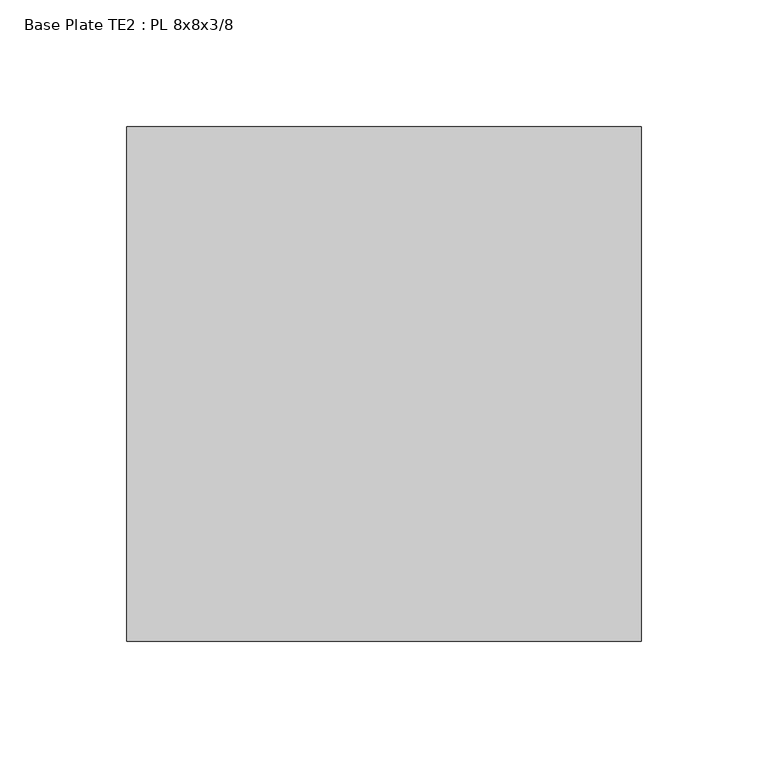
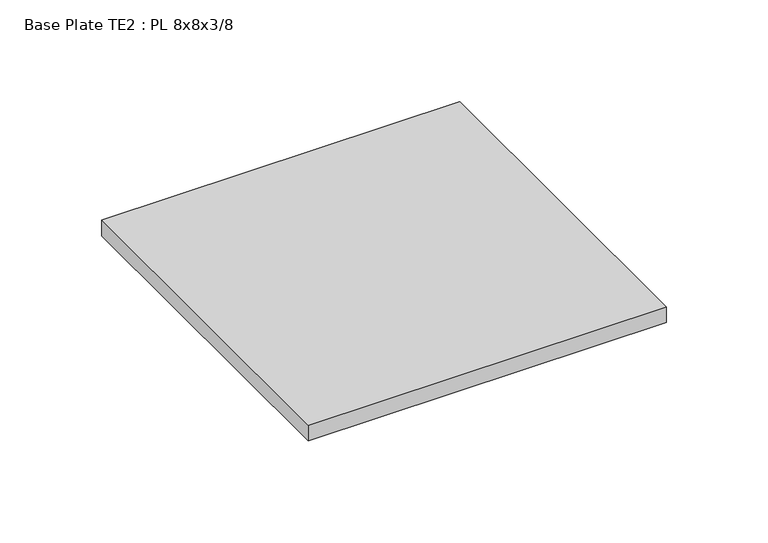
"""IFC4 building model written with IfcOpenShell, lengths in millimetres: proxy geometry, Base Plate TE2 : PL 8x8x3/8."""

from ifc_helpers import new_model, si_unit, frame, origin, place, context, project, spatial, polyline, outline, extrude, source, transform, mapped, element, save


def base_plate_te2_pl_8x8x3_8_a4684d66(model_context):
    return source(origin(), model_context, "Body", "SweptSolid", [
        extrude(outline(polyline([(590318.6599233, -533941.0913841), (590318.6599233, -534144.2913841), (590115.4599233, -534144.2913841), (590115.4599233, -533941.0913841), (590318.6599233, -533941.0913841)])), frame((0.0, 0.0, 19.05), z_axis=(0.0, 0.0, 1.0), x_axis=(1.0, 0.0, 0.0)), (0.0, 0.0, 1.0), 9.525),
    ])


if __name__ == "__main__":
    model = new_model("IFC4")
    model_context = context("Model", 3, world=origin())
    ifc_project = project(units=[si_unit("LENGTHUNIT", "METRE", prefix="MILLI")], contexts=[model_context])
    site = spatial("IfcSite", under=ifc_project)
    building = spatial("IfcBuilding", under=site)
    placement = place(None, origin())
    base_plate_te2_pl_8x8x3_8_shape = base_plate_te2_pl_8x8x3_8_a4684d66(model_context)
    element("IfcBuildingElementProxy", 1, Name="Base Plate TE2 : PL 8x8x3/8", ObjectType="Base Plate TE2 : PL 8x8x3/8", at=placement, inside=building, context=model_context, shape_type="MappedRepresentation", body=[
        mapped(base_plate_te2_pl_8x8x3_8_shape, transform((0.0, 0.0, 0.0), x_axis=(1.0, 0.0, 0.0), y_axis=(0.0, 1.0, 0.0), z_axis=(0.0, 0.0, 1.0))),
    ])
    save(model, "model.ifc")

# Revit data of these elements
# Element 1 (IfcBuildingElementProxy, "Base Plate TE2 : PL 8x8x3/8")
#   Materials on its faces: "GALV. STL BASE PLATE"
# Materials
#   "GALV. STL BASE PLATE": class "Generic", colour RGB 211 211 207, transparency 0, Cost = 0
